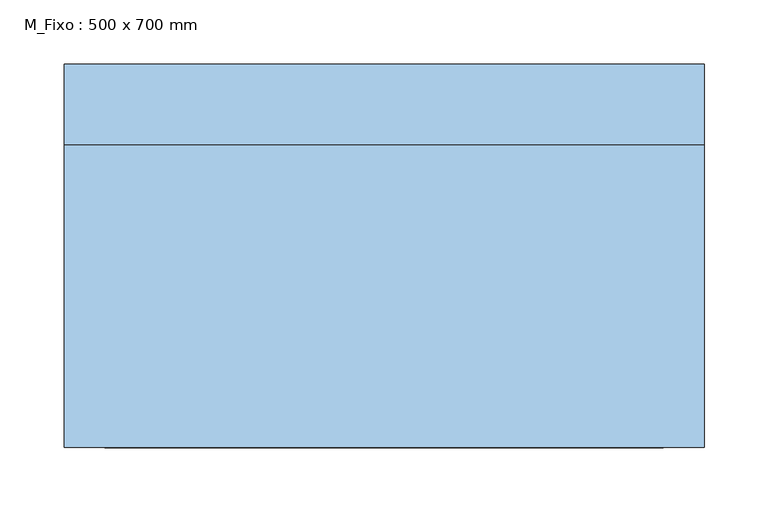
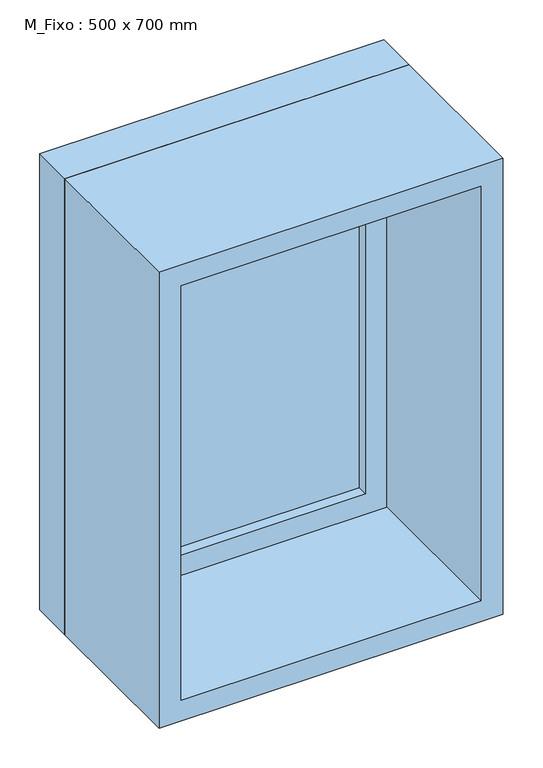
"""IFC4 building model written with IfcOpenShell, lengths in millimetres: window geometry, M_Fixo : 500 x 700 mm."""

from ifc_helpers import new_model, si_unit, frame, origin, place, context, project, spatial, polyline, outline, extrude, source, transform, mapped, element, save


def m_fixo_500_x_700_mm_b431b1bd(model_context):
    return source(origin(), model_context, "Body", "SweptSolid", [
        extrude(outline(polyline([(-187.0, 128.0), (187.0, 128.0), (187.0, 116.0), (-187.0, 116.0), (-187.0, 128.0)])), frame((0.0, 0.0, 978.0), z_axis=(0.0, 0.0, 1.0), x_axis=(1.0, 0.0, 0.0)), (0.0, 0.0, 1.0), 574.0),
        extrude(outline(polyline([(1596.0, -231.0), (934.0, -231.0), (934.0, 231.0), (1596.0, 231.0), (1596.0, -231.0)]), holes=[polyline([(1552.0, -187.0), (1552.0, 187.0), (978.0, 187.0), (978.0, -187.0), (1552.0, -187.0)])]), frame((0.0, 100.0, 0.0), z_axis=(0.0, 1.0, 0.0), x_axis=(0.0, 0.0, 1.0)), (0.0, 0.0, 1.0), 44.0),
        extrude(outline(polyline([(1615.0, -250.0), (915.0, -250.0), (915.0, 250.0), (1615.0, 250.0), (1615.0, -250.0)]), holes=[polyline([(1596.0, -231.0), (1596.0, 231.0), (934.0, 231.0), (934.0, -231.0), (1596.0, -231.0)])]), frame((0.0, 100.0, 0.0), z_axis=(0.0, 1.0, 0.0), x_axis=(0.0, 0.0, 1.0)), (0.0, 0.0, 1.0), 63.0),
        extrude(outline(polyline([(1615.0, -250.0), (915.0, -250.0), (915.0, 250.0), (1615.0, 250.0), (1615.0, -250.0)]), holes=[polyline([(1583.0, -218.0), (1583.0, 218.0), (947.0, 218.0), (947.0, -218.0), (1583.0, -218.0)])]), frame((0.0, -137.0, 0.0), z_axis=(0.0, 1.0, 0.0), x_axis=(0.0, 0.0, 1.0)), (0.0, 0.0, 1.0), 237.0),
    ])


if __name__ == "__main__":
    model = new_model("IFC4")
    model_context = context("Model", 3, world=origin())
    ifc_project = project(units=[si_unit("LENGTHUNIT", "METRE", prefix="MILLI")], contexts=[model_context])
    site = spatial("IfcSite", under=ifc_project)
    building = spatial("IfcBuilding", under=site)
    placement = place(None, origin())
    m_fixo_500_x_700_mm_shape = m_fixo_500_x_700_mm_b431b1bd(model_context)
    element("IfcWindow", 1, ObjectType="M_Fixo : 500 x 700 mm", at=placement, inside=building, context=model_context, shape_type="MappedRepresentation", body=[
        mapped(m_fixo_500_x_700_mm_shape, transform((0.0, 0.0, 0.0), x_axis=(1.0, 0.0, 0.0), y_axis=(0.0, 1.0, 0.0), z_axis=(0.0, 0.0, 1.0))),
    ])
    save(model, "model.ifc")

# Revit data of these elements
# Type "M_Fixo : 500 x 700 mm"
#   Type Mark = "19"
#   Construction Type Id = "GSP4R"
#   Analytic Construction = "Vidraça única Pilkington 1/8 pol"
#   Visual Light Transmittance = 0.9
#   Thermal Resistance (R) = 0.271106 (m²·K)/W
#   Solar Heat Gain Coefficient = 0.78
#   Heat Transfer Coefficient (U) = 3.6886 W/(m²·K)
#   Height = 0.700 m
#   Altura-padrão do peitoril = 0.915 m
#   Width = 0.500 m
#   Janela aplicada = 0.019 m
#   Define Thermal Properties by = 1
#   Material da estrutura externa = Caixilho
#   Material da estrutura interna = Caixilho
#   Material do painel de vidro = Vidro
#   Caixilho = Caixilho
#   Wall Closure = (empty or 0)
# Element 1 (IfcWindow, "M_Fixo : 500 x 700 mm")
#   Materials on its faces: "Caixilho", "Vidro"
# Materials
#   "Caixilho": class "Madeira", colour RGB 224 178 126, transparency 0, Cost = 0
#   "Vidro": class "Vidro", colour RGB 0 128 192, transparency 0.9, Description = "Vidro de sílica", Cost = 0
